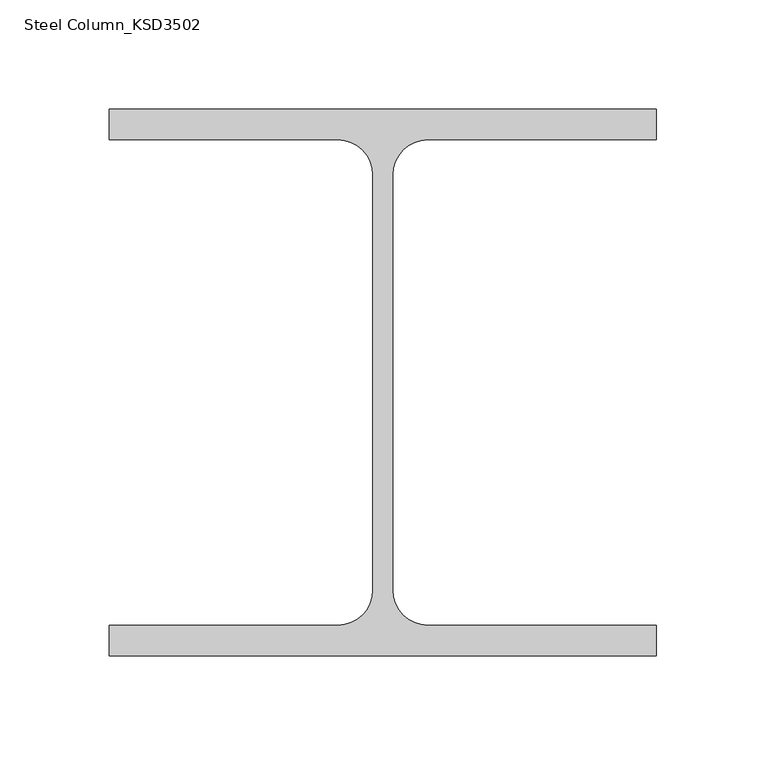
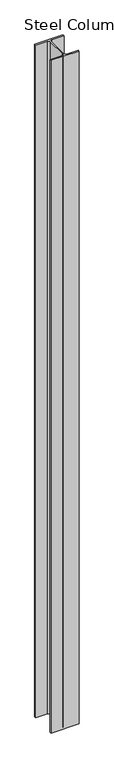
"""IFC4 building model written with IfcOpenShell, lengths in millimetres: column geometry, Steel Column_KSD3502 : H_SC_ASC_H-250×250x9x14."""

from ifc_helpers import new_model, si_unit, point, frame, frame_2d, origin, place, context, project, spatial, polyline, circle_curve, trimmed, segment, composite_curve, outline, extrude, source, transform, mapped, element, save


def steel_column_ksd3502_a4b71116(model_context):
    return source(origin(), model_context, "Body", "SweptSolid", [
        extrude(outline(composite_curve([segment(polyline([(125.0, 125.0), (125.0, 111.0), (20.5, 111.0)]), True, "CONTINUOUS"), segment(trimmed(circle_curve(frame_2d((20.5, 95.0)), 16.0), [point((20.5, 111.0))], [point((4.5, 95.0))], True, "CARTESIAN"), True, "CONTINUOUS"), segment(polyline([(4.5, 95.0), (4.5, -95.0)]), True, "CONTINUOUS"), segment(trimmed(circle_curve(frame_2d((20.5, -95.0)), 16.0), [point((4.5, -95.0))], [point((20.5, -111.0))], True, "CARTESIAN"), True, "CONTINUOUS"), segment(polyline([(20.5, -111.0), (125.0, -111.0), (125.0, -125.0), (-125.0, -125.0), (-125.0, -111.0), (-20.5, -111.0)]), True, "CONTINUOUS"), segment(trimmed(circle_curve(frame_2d((-20.5, -95.0)), 16.0), [point((-20.5, -111.0))], [point((-4.5, -95.0))], True, "CARTESIAN"), True, "CONTINUOUS"), segment(polyline([(-4.5, -95.0), (-4.5, 95.0)]), True, "CONTINUOUS"), segment(trimmed(circle_curve(frame_2d((-20.5, 95.0)), 16.0), [point((-4.5, 95.0))], [point((-20.5, 111.0))], True, "CARTESIAN"), True, "CONTINUOUS"), segment(polyline([(-20.5, 111.0), (-125.0, 111.0), (-125.0, 125.0), (125.0, 125.0)]), True, "CONTINUOUS")], self_intersect=False)), frame((0.0, 0.0, 599.9720055), z_axis=(0.0, 0.0, 1.0), x_axis=(1.0, 0.0, 0.0)), (0.0, 0.0, 1.0), 6300.0),
    ])


if __name__ == "__main__":
    model = new_model("IFC4")
    model_context = context("Model", 3, world=origin())
    ifc_project = project(units=[si_unit("LENGTHUNIT", "METRE", prefix="MILLI")], contexts=[model_context])
    site = spatial("IfcSite", under=ifc_project)
    building = spatial("IfcBuilding", under=site)
    placement = place(None, origin())
    steel_column_ksd3502_shape = steel_column_ksd3502_a4b71116(model_context)
    element("IfcColumn", 1, ObjectType="Steel Column_KSD3502 : H_SC_ASC_H-250×250x9x14", at=placement, inside=building, context=model_context, shape_type="MappedRepresentation", body=[
        mapped(steel_column_ksd3502_shape, transform((0.0, 0.0, 0.0), x_axis=(1.0, 0.0, 0.0), y_axis=(0.0, 1.0, 0.0), z_axis=(0.0, 0.0, 1.0))),
    ])
    save(model, "model.ifc")

# Revit data of these elements
# Type "Steel Column_KSD3502 : H_SC_ASC_H-250×250x9x14"
#   Width = 25.0 cm
#   Web Thickness = 0.9 cm
#   Web Fillet = 1.6 cm
#   Warping Constant = 507646.0 cm⁶
#   Torsional Moment of Inertia = 51.4681 cm⁴
#   Section Area = 92.18 cm²
#   Plastic Modulus weak axis = 444.0 cm³
#   Plastic Modulus strong axis = 960.0 cm³
#   Perimeter = 1.27 m²/m
#   Nominal Weight = 72.40 kgf/m
#   Moment of Inertia weak axis = 3650.00 cm⁴
#   Moment of Inertia strong axis = 10800.00 cm⁴
#   Height = 25.0 cm
#   Flange Thickness = 1.4 cm
#   Elastic Modulus weak axis = 292.0 cm³
#   Elastic Modulus strong axis = 867.0 cm³
#   Centroid Vertical = 12.5 cm
#   Centroid Horizontal = 12.5 cm
#   Bolt Spacing = 13.97 cm
#   Structural Material [instance default] = Steel, 45-345
#   Section Name Key = ""
#   Assembly Code = ""
# Element 1 (IfcColumn, "Steel Column_KSD3502 : H_SC_ASC_H-250×250x9x14")
#   Structural Material = A03AD029-00005_Anchor Bolt (Installation only)_M24
#   Materials on its faces: "A03AD029-00005_Anchor Bolt (Installation only)_M24"
# Materials
#   "Steel, 45-345": class "Metal", colour RGB 189 187 185, transparency 0, Description = "Steel 345 MPa", Cost = 0
#   "A03AD029-00005_Anchor Bolt (Installation only)_M24": class "Unassigned", colour RGB 84 83 81, transparency 0, Cost = 0
